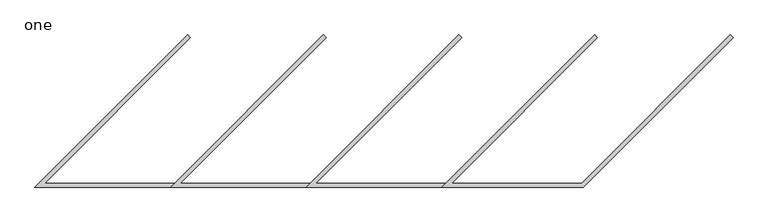
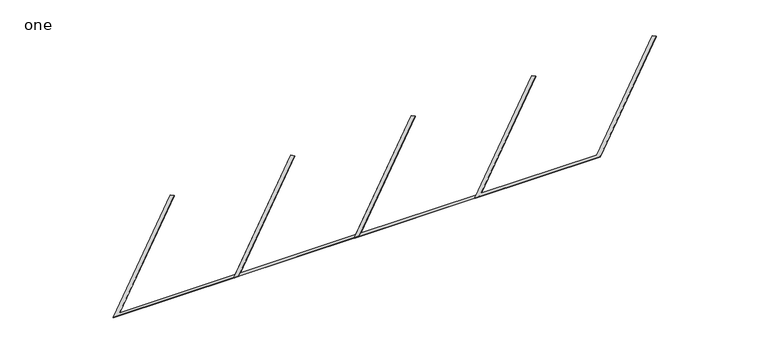
"""IFC4 building model written with IfcOpenShell, lengths in millimetres: proxy geometry, 321723 - Pavement Markings - Parking - Angled : one."""

from ifc_helpers import new_model, si_unit, origin, origin_with_axes, place, context, project, spatial, polyline, outline, extrude, source, transform, mapped, element, save


def one_61f29bb9(model_context):
    return source(origin(), model_context, "Body", "SweptSolid", [
        extrude(outline(polyline([(10345.2550515, 0.0), (14224.7256958, 3879.4706443), (14296.5677447, 3807.6285953), (10590.5391494, 101.6), (13895.273402, 101.6), (17673.1440463, 3879.4706443), (17744.9860952, 3807.6285953), (13937.3574999, 0.0), (10345.2550515, 0.0)])), origin_with_axes(), (0.0, 0.0, 1.0), 12.1533655),
        extrude(outline(polyline([(6896.836701, 0.0), (10776.3073453, 3879.4706443), (10848.1493943, 3807.6285953), (7142.1207989, 101.6), (10446.8550515, 101.6), (14224.7256958, 3879.4706443), (14296.5677447, 3807.6285953), (10488.9391494, 0.0), (6896.836701, 0.0)])), origin_with_axes(), (0.0, 0.0, 1.0), 12.1533655),
        extrude(outline(polyline([(3448.4183505, 0.0), (7327.8889948, 3879.4706443), (7399.7310438, 3807.6285953), (3693.7024484, 101.6), (6998.436701, 101.6), (10776.3073453, 3879.4706443), (10848.1493943, 3807.6285953), (7040.5207989, 0.0), (3448.4183505, 0.0)])), origin_with_axes(), (0.0, 0.0, 1.0), 12.1533655),
        extrude(outline(polyline([(0.0, 0.0), (3879.4706443, 3879.4706443), (3951.3126933, 3807.6285953), (245.2840979, 101.6), (3550.0183505, 101.6), (7327.8889948, 3879.4706443), (7399.7310438, 3807.6285953), (3592.1024484, 0.0), (0.0, 0.0)])), origin_with_axes(), (0.0, 0.0, 1.0), 12.1533655),
    ])


if __name__ == "__main__":
    model = new_model("IFC4")
    model_context = context("Model", 3, world=origin())
    ifc_project = project(units=[si_unit("LENGTHUNIT", "METRE", prefix="MILLI")], contexts=[model_context])
    site = spatial("IfcSite", under=ifc_project)
    building = spatial("IfcBuilding", under=site)
    placement = place(None, origin())
    one_shape = one_61f29bb9(model_context)
    element("IfcBuildingElementProxy", 1, Name="321723 - Pavement Markings - Parking - Angled : one", ObjectType="321723 - Pavement Markings - Parking - Angled : one", at=placement, inside=building, context=model_context, shape_type="MappedRepresentation", body=[
        mapped(one_shape, transform((0.0, 0.0, 0.0), x_axis=(1.0, 0.0, 0.0), y_axis=(0.0, 1.0, 0.0), z_axis=(0.0, 0.0, 1.0))),
    ])
    save(model, "model.ifc")

# Revit data of these elements
# Type "321723 - Pavement Markings - Parking - Angled : one"
#   Type Mark = "P1"
#   run [instance default] = 46' - 4.22888"
#   Width_Host = 8' - 0"
#   Offset = 11' - 3.7645"
#   Length_Host = 18' - 0"
#   Angle_Host = 45.00°
#   Parking_Count [instance default] = 4
